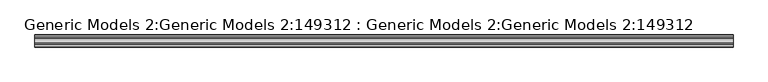
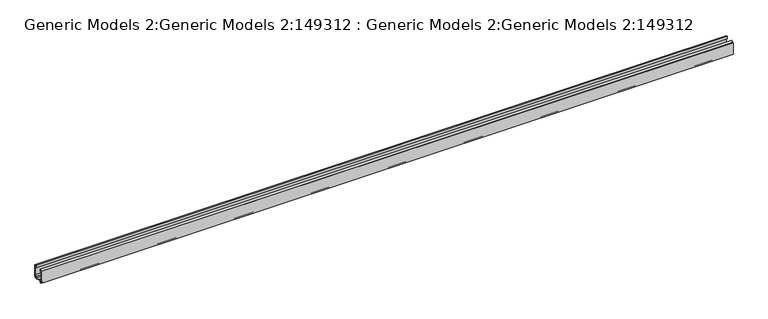
"""IFC4 building model written with IfcOpenShell, lengths in millimetres: proxy geometry, Generic Models 2:Generic Models 2:149312 : Generic Models 2:Generic Models 2:149312."""

from ifc_helpers import new_model, si_unit, frame, origin, place, context, project, spatial, polyline, outline, extrude, source, transform, mapped, element, save


def generic_models_2_generic_models_2_149312_generic_models_2_389c60cf(model_context):
    return source(origin(), model_context, "Body", "SweptSolid", [
        extrude(outline(polyline([(-10.4561158, 58.6381886), (-10.4561158, 73.2908075), (-0.4974764, 71.0720433), (-0.4974764, 68.9706283), (-7.4216914, 69.5530389), (-7.4216914, 64.1127391), (-5.4980393, 63.7843107), (-5.4980393, 65.8225741), (-4.4736904, 65.8225741), (-3.6336448, 64.0210905), (-3.6336448, 61.940792), (-4.4940931, 60.4504517), (-5.58328, 60.4504517), (-5.58328, 62.7048399), (-7.4216914, 60.8664286), (-7.4216914, 58.6381886), (-10.4561158, 58.6381886)])), frame((0.0, 0.0, 0.0), z_axis=(1.0, 0.0, 0.0), x_axis=(0.0, 1.0, 0.0)), (0.0, 0.0, 1.0), 3657.6),
        extrude(outline(polyline([(-2.5494865, 15.7119514), (-2.5494865, 58.6381886), (-7.1148459, 58.6381886), (-7.1148459, 60.6837832), (-5.8105155, 61.9881137), (-5.8105155, 60.1797386), (-4.3281979, 60.1797386), (-3.3343776, 61.9010859), (-3.3343776, 64.182505), (-4.2197993, 66.081298), (-5.8104575, 66.081298), (-5.8104575, 64.0480745), (-7.1148459, 64.270775), (-7.1148459, 69.3104575), (0.0, 68.7120125), (0.0, 6.2847806), (-3.557423, 6.2847806), (-3.557423, 0.0), (-5.573296, 0.0), (-5.573296, 6.2847806), (-16.4827264, 6.2847806), (-16.4827264, 0.0), (-18.4985994, 0.0), (-18.4985994, 6.2847806), (-49.56676, 6.2847806), (-49.56676, 0.0), (-51.5826331, 0.0), (-51.5826331, 6.2847806), (-60.1797386, 6.2847806), (-60.1797386, 7.6484594), (-59.3496732, 8.1820728), (-58.4010271, 7.5298786), (-51.5826331, 7.5298786), (-50.2782446, 8.834267), (-46.5429505, 8.834267), (-46.5429505, 14.1704015), (-60.0018674, 14.1704015), (-60.0018674, 15.7119514), (-44.5270775, 15.7119514), (-44.5270775, 8.834267), (-18.6171802, 8.834267), (-18.6171802, 15.7119514), (-2.5494865, 15.7119514)]), holes=[polyline([(-16.4827264, 8.4192344), (-3.1423903, 8.4192344), (-3.1423903, 14.1704015), (-16.4827264, 14.1704015), (-16.4827264, 8.4192344)])]), frame((0.0, 0.0, 0.0), z_axis=(1.0, 0.0, 0.0), x_axis=(0.0, 1.0, 0.0)), (0.0, 0.0, 1.0), 3657.6),
        extrude(outline(polyline([(-61.8875613, 70.6939849), (-61.8875613, 71.732598), (-50.4597811, 74.7946625), (-50.4597811, 63.1753705), (-56.5493952, 57.926704), (-57.7546992, 57.926704), (-57.7546992, 62.4558402), (-59.2967361, 66.670741), (-57.7546992, 66.9277471), (-57.7546992, 70.6939849), (-61.8875613, 70.6939849)])), frame((0.0, 0.0, 0.0), z_axis=(1.0, 0.0, 0.0), x_axis=(0.0, 1.0, 0.0)), (0.0, 0.0, 1.0), 3657.6),
        extrude(outline(polyline([(-58.1045752, 9.5621915), (-57.2450958, 9.0855634), (-57.1958513, 8.1356945), (-57.9364063, 7.6419912), (-58.949733, 8.3006536), (-60.3576097, 8.3006536), (-60.3576097, 5.9883287), (-63.5, 5.9883287), (-63.5, 70.4962652), (-58.0452848, 70.4962652), (-58.0452848, 67.3538749), (-59.8239963, 67.057423), (-58.0452848, 62.1956116), (-58.0452848, 57.926704), (-60.3576097, 57.926704), (-60.3576097, 13.3996265), (-48.2030812, 13.3996265), (-48.2030812, 12.0274777), (-58.1045752, 10.6129785), (-58.1045752, 9.5621915)])), frame((0.0, 0.0, 0.0), z_axis=(1.0, 0.0, 0.0), x_axis=(0.0, 1.0, 0.0)), (0.0, 0.0, 1.0), 3657.6),
    ])


if __name__ == "__main__":
    model = new_model("IFC4")
    model_context = context("Model", 3, world=origin())
    ifc_project = project(units=[si_unit("LENGTHUNIT", "METRE", prefix="MILLI")], contexts=[model_context])
    site = spatial("IfcSite", under=ifc_project)
    building = spatial("IfcBuilding", under=site)
    placement = place(None, origin())
    generic_models_2_generic_models_2_149312_generic_models_2_shape = generic_models_2_generic_models_2_149312_generic_models_2_389c60cf(model_context)
    element("IfcBuildingElementProxy", 1, Name="Generic Models 2:Generic Models 2:149312 : Generic Models 2:Generic Models 2:149312", ObjectType="Generic Models 2:Generic Models 2:149312 : Generic Models 2:Generic Models 2:149312", at=placement, inside=building, context=model_context, shape_type="MappedRepresentation", body=[
        mapped(generic_models_2_generic_models_2_149312_generic_models_2_shape, transform((0.0, 0.0, 0.0), x_axis=(1.0, 0.0, 0.0), y_axis=(0.0, 1.0, 0.0), z_axis=(0.0, 0.0, 1.0))),
    ])
    save(model, "model.ifc")

# Revit data of these elements
# Project information
#   IfcSite GUID = "1HspfKvnb2I8J8j3XW2lMe"
#   IfcBuilding GUID = "1HspfKvnb2I8J8j3XW2lMh"
#   IfcProject GUID = "1HspfKvnb2I8J8j3XW2lMg"
#   NumberOfStoreys = "1"
#   NameOverride = "Default"
#   Project Issue Date = "Issue Date"
#   Project Status = "Project Status"
#   Client Name = "Owner"
#   Project Address = "Enter address here"
#   Project Name = "PROJECT NAME"
#   Project Number = "Project Number"
# Type "Generic Models 2:Generic Models 2:149312 : Generic Models 2:Generic Models 2:149312"
#   NameOverride = "Generic Models 2:Generic Models 2:149312"
#   ObjectTypeOverride = "Generic Models 2"
#   Reference = "Generic Models 2"
#   Tag = "149312"
# Element 1 (IfcBuildingElementProxy, "Generic Models 2:Generic Models 2:149312 : Generic Models 2:Generic Models 2:149312")
#   Materials on its faces: "THERMAL BROKEN ALUMINUM STOREFRONT FOR POLYCARBONATE"
# Materials
#   "THERMAL BROKEN ALUMINUM STOREFRONT FOR POLYCARBONATE": class "Unassigned", colour RGB 244 244 244, transparency 0
